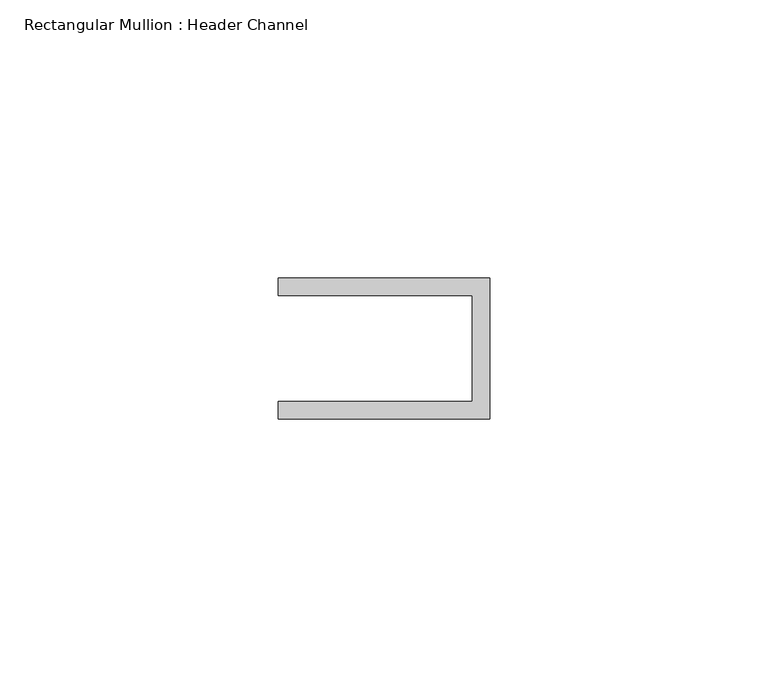
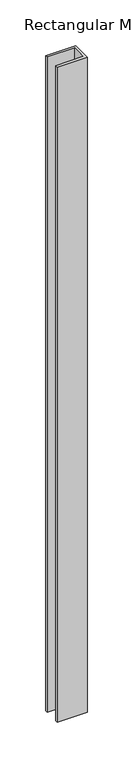
"""IFC4 building model written with IfcOpenShell, lengths in millimetres: member geometry, Rectangular Mullion : Header Channel."""

from ifc_helpers import new_model, si_unit, frame, origin, place, context, project, spatial, polyline, outline, extrude, source, transform, mapped, element, save


def rectangular_mullion_header_channel_cdd7834f(model_context):
    return source(origin(), model_context, "Body", "SweptSolid", [
        extrude(outline(polyline([(0.0, 12.7), (0.0, -12.7), (-38.1, -12.7), (-38.1, -9.525), (-3.175, -9.525), (-3.175, 9.525), (-38.1, 9.525), (-38.1, 12.7), (0.0, 12.7)])), frame((0.0, 0.0, -877.8875), z_axis=(0.0, 0.0, 1.0), x_axis=(1.0, 0.0, 0.0)), (0.0, 0.0, 1.0), 877.8875),
    ])


if __name__ == "__main__":
    model = new_model("IFC4")
    model_context = context("Model", 3, world=origin())
    ifc_project = project(units=[si_unit("LENGTHUNIT", "METRE", prefix="MILLI")], contexts=[model_context])
    site = spatial("IfcSite", under=ifc_project)
    building = spatial("IfcBuilding", under=site)
    placement = place(None, origin())
    rectangular_mullion_header_channel_shape = rectangular_mullion_header_channel_cdd7834f(model_context)
    element("IfcMember", 1, ObjectType="Rectangular Mullion : Header Channel", at=placement, inside=building, context=model_context, shape_type="MappedRepresentation", body=[
        mapped(rectangular_mullion_header_channel_shape, transform((0.0, 0.0, 0.0), x_axis=(1.0, 0.0, 0.0), y_axis=(0.0, 1.0, 0.0), z_axis=(0.0, 0.0, 1.0))),
    ])
    save(model, "model.ifc")

# Revit data of these elements
# Type "Rectangular Mullion : Header Channel"
#   built-in parameter 1007322 = 0.0833333 (stored number, unit not read)
#   built-in parameter 1007321 = -0.03125 (stored number, unit not read)
#   built-in parameter 1007320 = 0.0416667 (stored number, unit not read)
# Element 1 (IfcMember, "Rectangular Mullion : Header Channel")
#   Materials on its faces: "ALUM"
# Materials
#   "ALUM": class "Generic", colour RGB 157 157 157, transparency 0, Cost = 0
